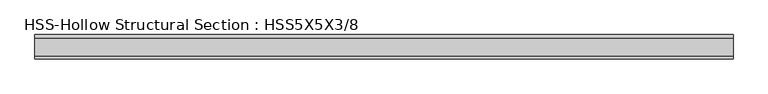
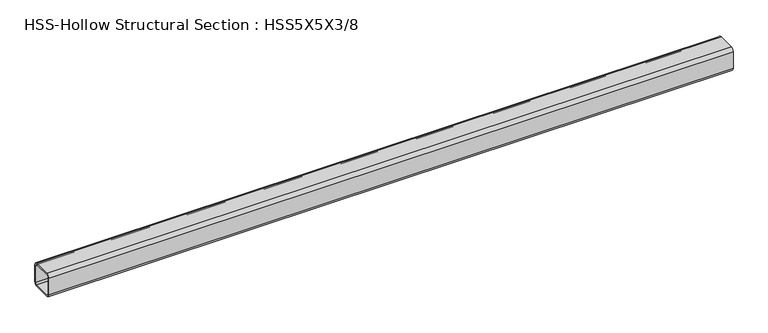
"""IFC4 building model written with IfcOpenShell, lengths in millimetres: member geometry, HSS-Hollow Structural Section : HSS5X5X3/8."""

from ifc_helpers import new_model, si_unit, point, frame, frame_2d, origin, place, context, project, spatial, polyline, circle_curve, trimmed, segment, composite_curve, outline, extrude, source, transform, mapped, element, save


def hss_hollow_structural_section_hss5x5x3_8_60919f1c(model_context):
    return source(origin(), model_context, "Body", "SweptSolid", [
        extrude(outline(composite_curve([segment(polyline([(63.5, 45.7708), (63.5, -45.7708)]), True, "CONTINUOUS"), segment(trimmed(circle_curve(frame_2d((45.7708, -45.7708)), 17.7292), [point((63.5, -45.7708))], [point((45.7708, -63.5))], False, "CARTESIAN"), True, "CONTINUOUS"), segment(polyline([(45.7708, -63.5), (-45.7708, -63.5)]), True, "CONTINUOUS"), segment(trimmed(circle_curve(frame_2d((-45.7708, -45.7708)), 17.7292), [point((-45.7708, -63.5))], [point((-63.5, -45.7708))], False, "CARTESIAN"), True, "CONTINUOUS"), segment(polyline([(-63.5, -45.7708), (-63.5, 45.7708)]), True, "CONTINUOUS"), segment(trimmed(circle_curve(frame_2d((-45.7708, 45.7708)), 17.7292), [point((-63.5, 45.7708))], [point((-45.7708, 63.5))], False, "CARTESIAN"), True, "CONTINUOUS"), segment(polyline([(-45.7708, 63.5), (45.7708, 63.5)]), True, "CONTINUOUS"), segment(trimmed(circle_curve(frame_2d((45.7708, 45.7708)), 17.7292), [point((45.7708, 63.5))], [point((63.5, 45.7708))], False, "CARTESIAN"), True, "CONTINUOUS")], self_intersect=False), holes=[composite_curve([segment(trimmed(circle_curve(frame_2d((-45.7708, 45.7708)), 8.8646), [point((-45.7708, 54.6354))], [point((-54.6354, 45.7708))], True, "CARTESIAN"), True, "CONTINUOUS"), segment(polyline([(-54.6354, 45.7708), (-54.6354, -45.7708)]), True, "CONTINUOUS"), segment(trimmed(circle_curve(frame_2d((-45.7708, -45.7708)), 8.8646), [point((-54.6354, -45.7708))], [point((-45.7708, -54.6354))], True, "CARTESIAN"), True, "CONTINUOUS"), segment(polyline([(-45.7708, -54.6354), (45.7708, -54.6354)]), True, "CONTINUOUS"), segment(trimmed(circle_curve(frame_2d((45.7708, -45.7708)), 8.8646), [point((45.7708, -54.6354))], [point((54.6354, -45.7708))], True, "CARTESIAN"), True, "CONTINUOUS"), segment(polyline([(54.6354, -45.7708), (54.6354, 45.7708)]), True, "CONTINUOUS"), segment(trimmed(circle_curve(frame_2d((45.7708, 45.7708)), 8.8646), [point((54.6354, 45.7708))], [point((45.7708, 54.6354))], True, "CARTESIAN"), True, "CONTINUOUS"), segment(polyline([(45.7708, 54.6354), (-45.7708, 54.6354)]), True, "CONTINUOUS")], self_intersect=False)]), frame((-1806.634118, 0.0, 0.0), z_axis=(1.0, 0.0, 0.0), x_axis=(0.0, 1.0, 0.0)), (0.0, 0.0, 1.0), 3613.268236),
    ])


if __name__ == "__main__":
    model = new_model("IFC4")
    model_context = context("Model", 3, world=origin())
    ifc_project = project(units=[si_unit("LENGTHUNIT", "METRE", prefix="MILLI")], contexts=[model_context])
    site = spatial("IfcSite", under=ifc_project)
    building = spatial("IfcBuilding", under=site)
    placement = place(None, origin())
    hss_hollow_structural_section_hss5x5x3_8_shape = hss_hollow_structural_section_hss5x5x3_8_60919f1c(model_context)
    element("IfcMember", 1, ObjectType="HSS-Hollow Structural Section : HSS5X5X3/8", at=placement, inside=building, context=model_context, shape_type="MappedRepresentation", body=[
        mapped(hss_hollow_structural_section_hss5x5x3_8_shape, transform((0.0, 0.0, 0.0), x_axis=(1.0, 0.0, 0.0), y_axis=(0.0, 1.0, 0.0), z_axis=(0.0, 0.0, 1.0))),
    ])
    save(model, "model.ifc")

# Revit data of these elements
# Type "HSS-Hollow Structural Section : HSS5X5X3/8"
#   Assembly Code = "B10"
#   Shape = "Square"
#   W = 22.3
#   Ht = 0' - 5"
#   Length [instance default] = 5' - 0"
#   b = 0' - 5"
#   kr = 0' - 0.698"
#   t = 0' - 0.349"
#   A = 0.0429167 SF
#   Structural Material [instance default] = Steel ASTM A500, Grade B, Rectangular and Square
# Element 1 (IfcMember, "HSS-Hollow Structural Section : HSS5X5X3/8")
#   Materials on its faces: "Steel ASTM A500, Grade B, Rectangular and Square"
# Materials
#   "Steel ASTM A500, Grade B, Rectangular and Square": class "Metal", colour RGB 199 199 199, transparency 0, Description = "Carbon steel", Cost = 0
